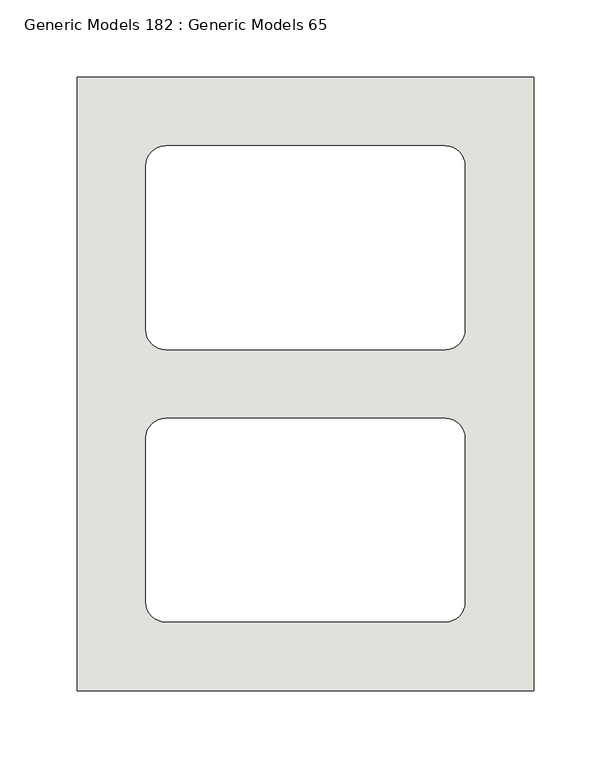
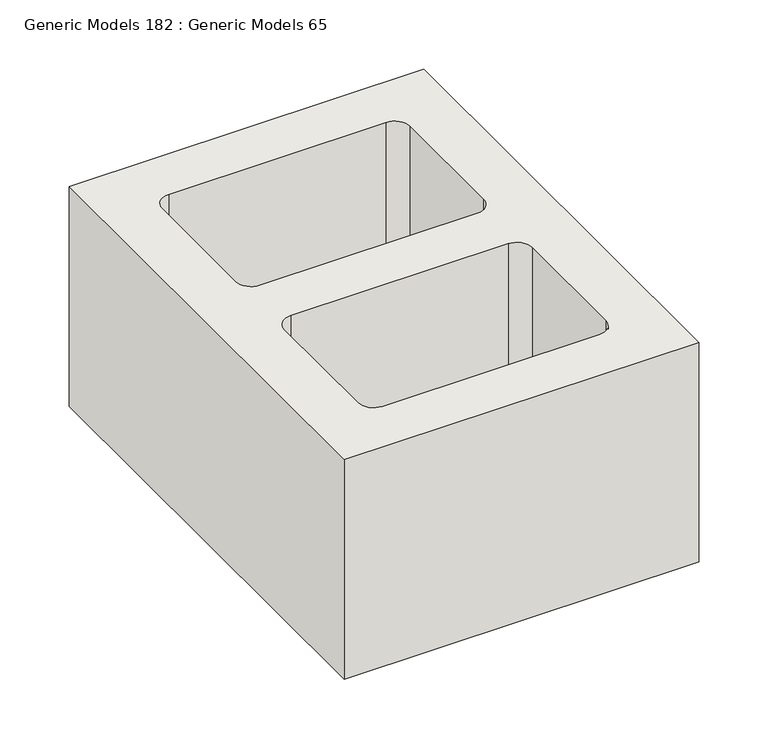
"""IFC4 building model written with IfcOpenShell, lengths in millimetres: wall geometry, Generic Models 182 : Generic Models 65."""

from ifc_helpers import new_model, si_unit, point, frame, frame_2d, origin, place, context, project, spatial, polyline, circle_curve, trimmed, segment, composite_curve, outline, extrude, source, transform, mapped, element, save


def generic_models_182_generic_models_65_5e5fb3b7(model_context):
    return source(origin(), model_context, "Body", "SweptSolid", [
        extrude(outline(polyline([(375249.9901825, 292.1), (374954.7151825, 292.1), (374954.7151825, 688.975), (375249.9901825, 688.975), (375249.9901825, 292.1)]), holes=[composite_curve([segment(polyline([(375205.5401825, 525.4625), (375205.5401825, 631.825)]), True, "CONTINUOUS"), segment(trimmed(circle_curve(frame_2d((375192.8401825, 631.825)), 12.7), [point((375205.5401825, 631.825))], [point((375192.8401825, 644.525))], True, "CARTESIAN"), True, "CONTINUOUS"), segment(polyline([(375192.8401825, 644.525), (375011.8651825, 644.525)]), True, "CONTINUOUS"), segment(trimmed(circle_curve(frame_2d((375011.8651825, 631.825)), 12.7), [point((375011.8651825, 644.525))], [point((374999.1651825, 631.825))], True, "CARTESIAN"), True, "CONTINUOUS"), segment(polyline([(374999.1651825, 631.825), (374999.1651825, 525.4625)]), True, "CONTINUOUS"), segment(trimmed(circle_curve(frame_2d((375011.8651825, 525.4625)), 12.7), [point((374999.1651825, 525.4625))], [point((375011.8651825, 512.7625))], True, "CARTESIAN"), True, "CONTINUOUS"), segment(polyline([(375011.8651825, 512.7625), (375192.8401825, 512.7625)]), True, "CONTINUOUS"), segment(trimmed(circle_curve(frame_2d((375192.8401825, 525.4625)), 12.7), [point((375192.8401825, 512.7625))], [point((375205.5401825, 525.4625))], True, "CARTESIAN"), True, "CONTINUOUS")], self_intersect=False), composite_curve([segment(polyline([(374999.1651825, 455.6125), (374999.1651825, 349.25)]), True, "CONTINUOUS"), segment(trimmed(circle_curve(frame_2d((375011.8651825, 349.25)), 12.7), [point((374999.1651825, 349.25))], [point((375011.8651825, 336.55))], True, "CARTESIAN"), True, "CONTINUOUS"), segment(polyline([(375011.8651825, 336.55), (375192.8401825, 336.55)]), True, "CONTINUOUS"), segment(trimmed(circle_curve(frame_2d((375192.8401825, 349.25)), 12.7), [point((375192.8401825, 336.55))], [point((375205.5401825, 349.25))], True, "CARTESIAN"), True, "CONTINUOUS"), segment(polyline([(375205.5401825, 349.25), (375205.5401825, 455.6125)]), True, "CONTINUOUS"), segment(trimmed(circle_curve(frame_2d((375192.8401825, 455.6125)), 12.7), [point((375205.5401825, 455.6125))], [point((375192.8401825, 468.3125))], True, "CARTESIAN"), True, "CONTINUOUS"), segment(polyline([(375192.8401825, 468.3125), (375011.8651825, 468.3125)]), True, "CONTINUOUS"), segment(trimmed(circle_curve(frame_2d((375011.8651825, 455.6125)), 12.7), [point((375011.8651825, 468.3125))], [point((374999.1651825, 455.6125))], True, "CARTESIAN"), True, "CONTINUOUS")], self_intersect=False)]), frame((0.0, 0.0, 1469.4712589), z_axis=(0.0, 0.0, 1.0), x_axis=(1.0, 0.0, 0.0)), (0.0, 0.0, 1.0), 193.675),
    ])


if __name__ == "__main__":
    model = new_model("IFC4")
    model_context = context("Model", 3, world=origin())
    ifc_project = project(units=[si_unit("LENGTHUNIT", "METRE", prefix="MILLI")], contexts=[model_context])
    site = spatial("IfcSite", under=ifc_project)
    building = spatial("IfcBuilding", under=site)
    placement = place(None, origin())
    generic_models_182_generic_models_65_shape = generic_models_182_generic_models_65_5e5fb3b7(model_context)
    element("IfcWall", 1, ObjectType="Generic Models 182 : Generic Models 65", at=placement, inside=building, context=model_context, shape_type="MappedRepresentation", body=[
        mapped(generic_models_182_generic_models_65_shape, transform((0.0, 0.0, 0.0), x_axis=(1.0, 0.0, 0.0), y_axis=(0.0, 1.0, 0.0), z_axis=(0.0, 0.0, 1.0))),
    ])
    save(model, "model.ifc")

# Revit data of these elements
# Element 1 (IfcWall, "Generic Models 182 : Generic Models 65")
#   Materials on its faces: "CMU (SEE 'WALL TAG' FOR SIZE)"
# Materials
#   "CMU (SEE 'WALL TAG' FOR SIZE)": class "Masonry", colour RGB 203 203 199, transparency 0, Description = "Concrete masonry units", Cost = 0
